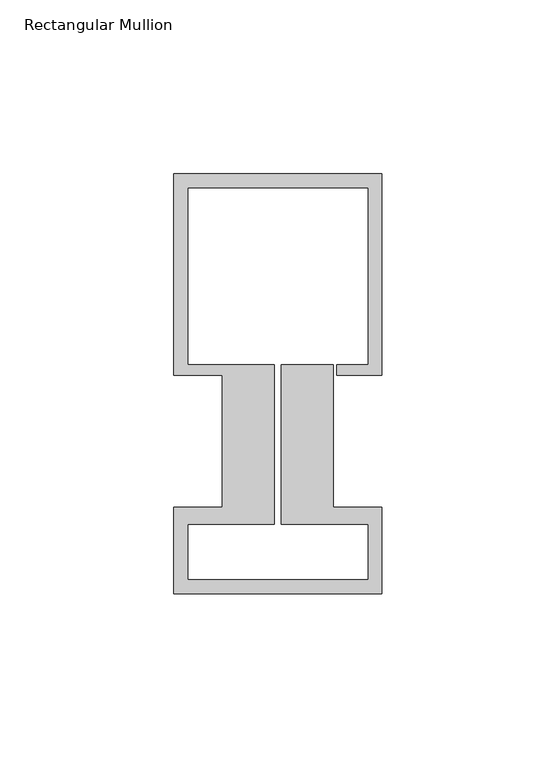
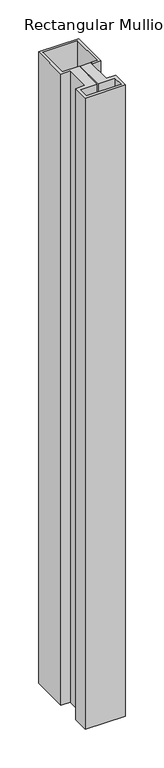
"""IFC4 building model written with IfcOpenShell, lengths in millimetres: member geometry, Rectangular Mullion : Schueco_FWS-60-SI_Tran_CovCap-20mm_Tran-55mm."""

from ifc_helpers import new_model, si_unit, frame, origin, place, context, project, spatial, polyline, outline, extrude, source, transform, mapped, element, save


def rectangular_mullion_96f2d495(model_context):
    return source(origin(), model_context, "Body", "SweptSolid", [
        extrude(outline(polyline([(-60.0, 96.0), (0.0, 96.0), (0.0, 38.0), (-13.0, 38.0), (-13.0, 41.0), (-4.0, 41.0), (-4.0, 92.0), (-56.0, 92.0), (-56.0, 41.0), (-31.0, 41.0), (-31.0, -5.0), (-56.0, -5.0), (-56.0, -21.0), (-4.0, -21.0), (-4.0, -5.0), (-29.0, -5.0), (-29.0, 41.0), (-14.0, 41.0), (-14.0, -0.1), (0.0, -0.1), (0.0, -25.0), (-60.0, -25.0), (-60.0, -0.1), (-46.0, -0.1), (-46.0, 38.0), (-60.0, 38.0), (-60.0, 96.0)])), frame((0.0, 0.0, -1000.0), z_axis=(0.0, 0.0, 1.0), x_axis=(1.0, 0.0, 0.0)), (0.0, 0.0, 1.0), 1000.0),
    ])


if __name__ == "__main__":
    model = new_model("IFC4")
    model_context = context("Model", 3, world=origin())
    ifc_project = project(units=[si_unit("LENGTHUNIT", "METRE", prefix="MILLI")], contexts=[model_context])
    site = spatial("IfcSite", under=ifc_project)
    building = spatial("IfcBuilding", under=site)
    placement = place(None, origin())
    rectangular_mullion_shape = rectangular_mullion_96f2d495(model_context)
    element("IfcMember", 1, ObjectType="Rectangular Mullion : Schueco_FWS-60-SI_Tran_CovCap-20mm_Tran-55mm", at=placement, inside=building, context=model_context, shape_type="MappedRepresentation", body=[
        mapped(rectangular_mullion_shape, transform((0.0, 0.0, 0.0), x_axis=(1.0, 0.0, 0.0), y_axis=(0.0, 1.0, 0.0), z_axis=(0.0, 0.0, 1.0))),
    ])
    save(model, "model.ifc")

# Revit data of these elements
# Type "Rectangular Mullion : Schueco_FWS-60-SI_Tran_CovCap-20mm_Tran-55mm"
#   Model = "FWS 60.SI"
#   Manufacturer = "Schueco International KG"
#   Type Comments = "Transom"
#   Schueco thermal insulation standard = "Suitable for passive houses"
#   Burglar resistance = "RC 3"
#   Thermal insulation = "to 0.70 W/(m²K)"
#   built-in parameter 1007322 = 0.396982 (stored number, unit not read)
#   built-in parameter 1007321 = 0.0524934 (stored number, unit not read)
#   built-in parameter 1007320 = 0.0524934 (stored number, unit not read)
# Element 1 (IfcMember, "Rectangular Mullion : Schueco_FWS-60-SI_Tran_CovCap-20mm_Tran-55mm")
#   Materials on its faces: "Alu"
# Materials
#   "Alu": class "Glas", colour RGB 140 140 140, transparency 0
